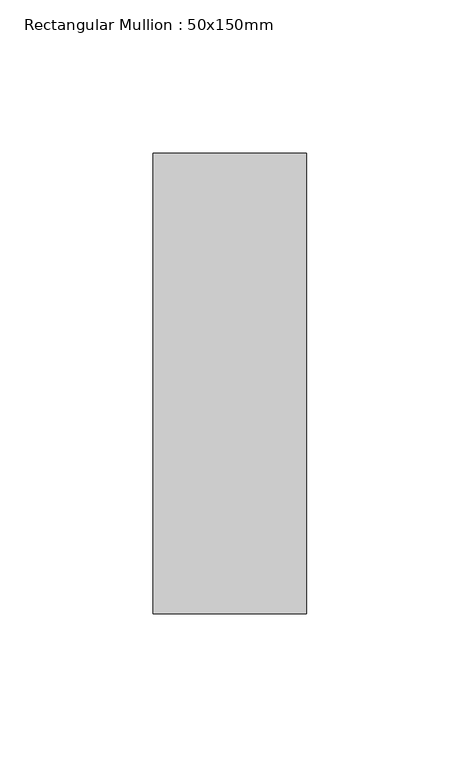
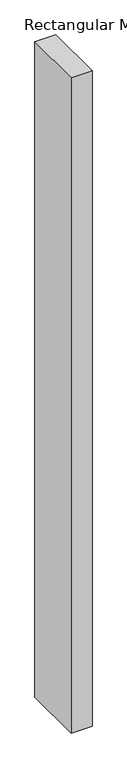
"""IFC4 building model written with IfcOpenShell, lengths in millimetres: member geometry, Rectangular Mullion : 50x150mm."""

from ifc_helpers import new_model, si_unit, frame, origin, place, context, project, spatial, polyline, outline, extrude, source, transform, mapped, element, save


def rectangular_mullion_50x150mm_fbedba44(model_context):
    return source(origin(), model_context, "Body", "SweptSolid", [
        extrude(outline(polyline([(0.0, 75.0), (0.0, -75.0), (-50.0, -75.0), (-50.0, 75.0), (0.0, 75.0)])), frame((0.0, 0.0, -1655.0000003), z_axis=(0.0, 0.0, 1.0), x_axis=(1.0, 0.0, 0.0)), (0.0, 0.0, 1.0), 1655.0000003),
    ])


if __name__ == "__main__":
    model = new_model("IFC4")
    model_context = context("Model", 3, world=origin())
    ifc_project = project(units=[si_unit("LENGTHUNIT", "METRE", prefix="MILLI")], contexts=[model_context])
    site = spatial("IfcSite", under=ifc_project)
    building = spatial("IfcBuilding", under=site)
    placement = place(None, origin())
    rectangular_mullion_50x150mm_shape = rectangular_mullion_50x150mm_fbedba44(model_context)
    element("IfcMember", 1, ObjectType="Rectangular Mullion : 50x150mm", at=placement, inside=building, context=model_context, shape_type="MappedRepresentation", body=[
        mapped(rectangular_mullion_50x150mm_shape, transform((0.0, 0.0, 0.0), x_axis=(1.0, 0.0, 0.0), y_axis=(0.0, 1.0, 0.0), z_axis=(0.0, 0.0, 1.0))),
    ])
    save(model, "model.ifc")

# Revit data of these elements
# Type "Rectangular Mullion : 50x150mm"
#   Keynote = "H11"
#   built-in parameter 1007304 = 0.492126 (stored number, unit not read)
#   built-in parameter 1007301 = 0.082021 (stored number, unit not read)
#   built-in parameter 1007300 = 0.082021 (stored number, unit not read)
# Element 1 (IfcMember, "Rectangular Mullion : 50x150mm")
#   Materials on its faces: "Aluminium"
# Materials
#   "Aluminium": class "Metal", colour RGB 247 247 247, transparency 0, Description = "Aluminium 6061", Cost = 0
